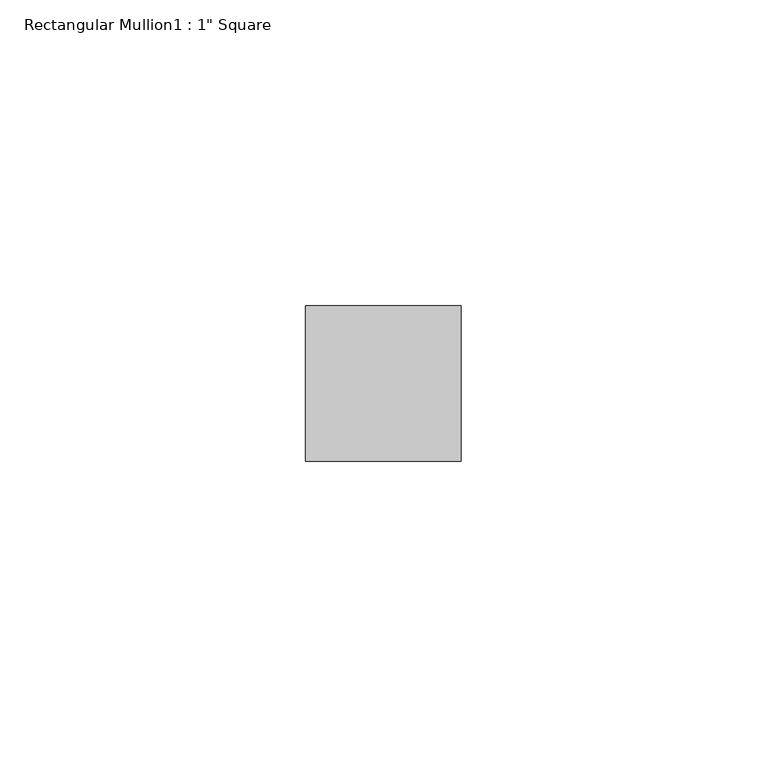
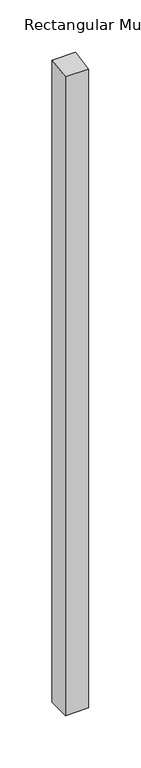
"""IFC4 building model written with IfcOpenShell, lengths in millimetres: member geometry."""

import ifcopenshell
import ifcopenshell.guid

model = None  # the IFC model being written
_history = None  # IfcOwnerHistory: only IFC2X3 demands one
_inside = {}  # id of a spatial element -> (the spatial element, [elements in it])
_under = {}  # id of a project, library or spatial element -> (it, [spatial elements below it])
_declared = {}  # id of a project -> (the project, [libraries it declares])
_typed = {}  # id of a type object -> (the type object, [elements of that type])
_made_of = {}  # id of a material, layer set ... -> (it, [elements and type objects made of it])


def new_model(schema):
    """Start an empty IFC model of exactly this schema.

    Asked for "IFC4X3", IfcOpenShell would pick the latest addendum, in which some entities
    have other attributes; the version numbers below select the first issue.
    IFC2X3 requires an IfcOwnerHistory on every rooted entity: one is made here for all.
    """
    global model, _history
    if schema == "IFC4X3":
        model = ifcopenshell.file(schema_version=(4, 3, 0, 0))
    else:
        model = ifcopenshell.file(schema=schema)
    _inside.clear()
    _under.clear()
    _declared.clear()
    _typed.clear()
    _made_of.clear()
    _history = None
    if model.schema == "IFC2X3":
        org = make("IfcOrganization", Name="unknown")
        user = make(
            "IfcPersonAndOrganization",
            ThePerson=make("IfcPerson", FamilyName="unknown"),
            TheOrganization=org,
        )
        app = make(
            "IfcApplication",
            ApplicationDeveloper=org,
            Version="unknown",
            ApplicationFullName="unknown",
            ApplicationIdentifier="unknown",
        )
        _history = make(
            "IfcOwnerHistory",
            OwningUser=user,
            OwningApplication=app,
            ChangeAction="ADDED",
            CreationDate=0,
        )
    return model


def make(cls, **values):
    """One entity of the class cls with the attributes given. An attribute that is None is left unset."""
    return model.create_entity(
        cls, **{name: value for name, value in values.items() if value is not None}
    )


def rooted(cls, **values):
    """An entity with a GlobalId (a new one), such as an element, a storey or a relation."""
    return make(cls, GlobalId=ifcopenshell.guid.new(), OwnerHistory=_history, **values)


def si_unit(unit_type, name, prefix=None):
    """IfcSIUnit, for example si_unit("LENGTHUNIT", "METRE", prefix="MILLI")."""
    return make("IfcSIUnit", UnitType=unit_type, Prefix=prefix, Name=name)


def assignment(units):
    """IfcUnitAssignment: the units of a project."""
    return None if units is None else make("IfcUnitAssignment", Units=units)


def point(xyz):
    """IfcCartesianPoint."""
    return None if xyz is None else make("IfcCartesianPoint", Coordinates=xyz)


def direction(xyz):
    """IfcDirection."""
    return None if xyz is None else make("IfcDirection", DirectionRatios=xyz)


def frame(location, z_axis=None, x_axis=None):
    """IfcAxis2Placement3D, a coordinate frame: its origin and axes. An axis left out is left unset."""
    return make(
        "IfcAxis2Placement3D",
        Location=point(location),
        Axis=direction(z_axis),
        RefDirection=direction(x_axis),
    )


def origin():
    """The frame at (0, 0, 0) with its axes left unset."""
    return frame((0.0, 0.0, 0.0))


def place(relative_to, where):
    """IfcLocalPlacement: puts the frame where relative to a parent placement (None: the world)."""
    return make(
        "IfcLocalPlacement", PlacementRelTo=relative_to, RelativePlacement=where
    )


def context(
    kind, dimensions, precision=None, world=None, true_north=None, identifier=None
):
    """IfcGeometricRepresentationContext, for example the 3D "Model" context."""
    return make(
        "IfcGeometricRepresentationContext",
        ContextIdentifier=identifier,
        ContextType=kind,
        CoordinateSpaceDimension=dimensions,
        Precision=precision,
        WorldCoordinateSystem=world,
        TrueNorth=true_north,
    )


def project(units=None, contexts=None):
    """IfcProject with its units and contexts."""
    return rooted(
        "IfcProject",
        Name="project",
        RepresentationContexts=contexts,
        UnitsInContext=assignment(units),
    )


def spatial(cls, under=None, at=None, **own):
    """A site, building, storey or space (cls), placed at a placement, below another one or the project."""
    s = rooted(cls, ObjectPlacement=at, **own)
    if under is not None:
        _under.setdefault(under.id(), (under, []))[1].append(s)
    return s


def polyline(points):
    """IfcPolyline through the points."""
    return make("IfcPolyline", Points=[point(p) for p in points])


def outline(outer, holes=None, kind="AREA"):
    """IfcArbitraryClosedProfileDef: a profile drawn as a closed curve; with holes, ...WithVoids."""
    if holes is None:
        return make("IfcArbitraryClosedProfileDef", ProfileType=kind, OuterCurve=outer)
    return make(
        "IfcArbitraryProfileDefWithVoids",
        ProfileType=kind,
        OuterCurve=outer,
        InnerCurves=holes,
    )


def extrude(swept, where, along, depth):
    """IfcExtrudedAreaSolid: the profile swept, set in the frame where, extruded along a direction by depth."""
    return make(
        "IfcExtrudedAreaSolid",
        SweptArea=swept,
        Position=where,
        ExtrudedDirection=direction(along),
        Depth=depth,
    )


def shape(context_of_items, identifier, shape_type, items):
    """IfcShapeRepresentation: the items that make up one representation, for example the "Body"."""
    return make(
        "IfcShapeRepresentation",
        ContextOfItems=context_of_items,
        RepresentationIdentifier=identifier,
        RepresentationType=shape_type,
        Items=items,
    )


def source(mapping_origin, context_of_items, identifier, shape_type, items):
    """IfcRepresentationMap: a shape defined once, which mapped items show again and again."""
    return make(
        "IfcRepresentationMap",
        MappingOrigin=mapping_origin,
        MappedRepresentation=shape(context_of_items, identifier, shape_type, items),
    )


def transform(
    local_origin,
    x_axis=None,
    y_axis=None,
    z_axis=None,
    scale=None,
    scale2=None,
    scale3=None,
    uniform=True,
):
    """IfcCartesianTransformationOperator3D, or its non-uniform kind. x_axis, y_axis, z_axis: its Axis1, 2, 3."""
    if uniform:
        return make(
            "IfcCartesianTransformationOperator3D",
            Axis1=direction(x_axis),
            Axis2=direction(y_axis),
            LocalOrigin=point(local_origin),
            Scale=scale,
            Axis3=direction(z_axis),
        )
    return make(
        "IfcCartesianTransformationOperator3DnonUniform",
        Axis1=direction(x_axis),
        Axis2=direction(y_axis),
        LocalOrigin=point(local_origin),
        Scale=scale,
        Axis3=direction(z_axis),
        Scale2=scale2,
        Scale3=scale3,
    )


def mapped(mapping_source, mapping_target):
    """IfcMappedItem: shows the shape of a source again, moved by a transform."""
    return make(
        "IfcMappedItem", MappingSource=mapping_source, MappingTarget=mapping_target
    )


def made_of(thing, what):
    """Note that an element or type object is made of a material, layer set ...; save() writes the relation."""
    if what is not None:
        _made_of.setdefault(what.id(), (what, []))[1].append(thing)
    return thing


def element(
    cls,
    number,
    at=None,
    inside=None,
    cuts=None,
    type_object=None,
    material=None,
    context=None,
    identifier="Body",
    shape_type=None,
    held_by="IfcProductDefinitionShape",
    body=None,
    shapes=None,
    **own,
):
    """One element of the class cls, such as IfcWall. Its Tag is "e" and its number.

    at: its placement. inside: the storey or other place that contains it. cuts: it is an
    opening in that element (IfcRelVoidsElement). A single representation is given by context,
    identifier, shape_type and body (its items); several are given by shapes. held_by: the class
    of the entity that holds the representations. save() writes the other relations.
    """
    e = rooted(cls, Tag="e%d" % number, ObjectPlacement=at, **own)
    if body is not None:
        shapes = [shape(context, identifier, shape_type, body)]
    if shapes is not None:
        e.Representation = make(held_by, Representations=shapes)
    if inside is not None:
        _inside.setdefault(inside.id(), (inside, []))[1].append(e)
    if cuts is not None:
        rooted(
            "IfcRelVoidsElement", RelatingBuildingElement=cuts, RelatedOpeningElement=e
        )
    if type_object is not None:
        _typed.setdefault(type_object.id(), (type_object, []))[1].append(e)
    return made_of(e, material)


def aggregate(whole, parts):
    """IfcRelAggregates: a whole, such as a stair, and the parts it consists of."""
    return rooted("IfcRelAggregates", RelatingObject=whole, RelatedObjects=parts)


def save(model, path):
    """Write the relations noted so far, then the file.

    IfcRelAggregates (storeys below a building ...), IfcRelContainedInSpatialStructure (elements
    in a storey), IfcRelDefinesByType, IfcRelAssociatesMaterial and IfcRelDeclares: one each for
    every whole, place, type object, material and project.
    """
    for whole, parts in _under.values():
        aggregate(whole, parts)
    for where, things in _inside.values():
        rooted(
            "IfcRelContainedInSpatialStructure",
            RelatedElements=things,
            RelatingStructure=where,
        )
    for kind, things in _typed.values():
        rooted("IfcRelDefinesByType", RelatedObjects=things, RelatingType=kind)
    for what, things in _made_of.values():
        rooted("IfcRelAssociatesMaterial", RelatedObjects=things, RelatingMaterial=what)
    for by, libraries in _declared.values():
        rooted("IfcRelDeclares", RelatingContext=by, RelatedDefinitions=libraries)
    model.write(path)


def member_6a737cc0(model_context):
    return source(origin(), model_context, "Body", "SweptSolid", [
        extrude(outline(polyline([(-44.45, -7.0452458), (-19.05, -3.019391), (-19.05, -749.7376951), (-44.45, -749.7376951), (-44.45, -7.0452458)])), frame((-12.7, 0.0, 0.0), z_axis=(1.0, 0.0, 0.0), x_axis=(0.0, 1.0, 0.0)), (0.0, 0.0, 1.0), 25.4),
    ])


if __name__ == "__main__":
    model = new_model("IFC4")
    model_context = context("Model", 3, world=origin())
    ifc_project = project(units=[si_unit("LENGTHUNIT", "METRE", prefix="MILLI")], contexts=[model_context])
    site = spatial("IfcSite", under=ifc_project)
    building = spatial("IfcBuilding", under=site)
    placement = place(None, origin())
    member_shape = member_6a737cc0(model_context)
    element("IfcMember", 1, ObjectType="Rectangular Mullion1 : 1\" Square", at=placement, inside=building, context=model_context, shape_type="MappedRepresentation", body=[
        mapped(member_shape, transform((0.0, 0.0, 0.0), x_axis=(1.0, 0.0, 0.0), y_axis=(0.0, 1.0, 0.0), z_axis=(0.0, 0.0, 1.0))),
    ])
    save(model, "model.ifc")

# Revit data of these elements
# Type "Rectangular Mullion1 : 1\" Square"
#   built-in parameter 1007351 = 0.104167 (stored number, unit not read)
#   built-in parameter 1007304 = 0.0833333 (stored number, unit not read)
#   built-in parameter 1007301 = 0.0416667 (stored number, unit not read)
#   built-in parameter 1007300 = 0.0416667 (stored number, unit not read)
